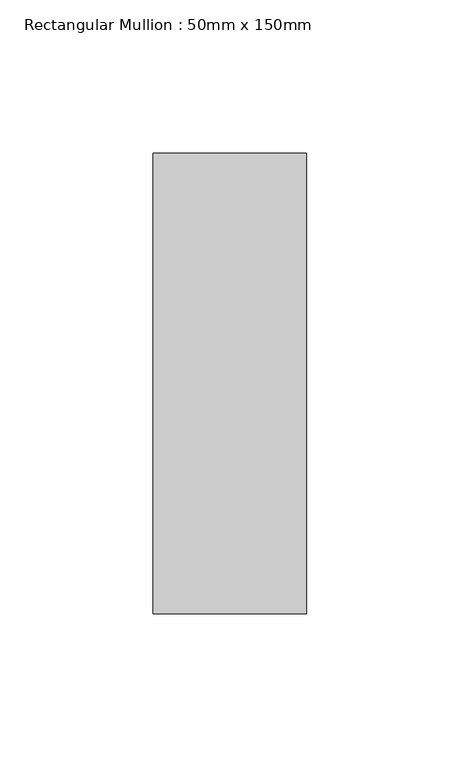
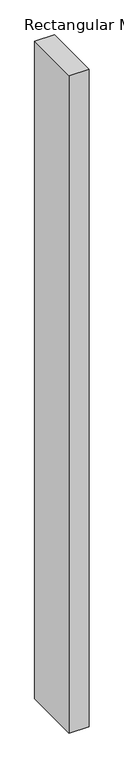
"""IFC4 building model written with IfcOpenShell, lengths in millimetres: member geometry, Rectangular Mullion : 50mm x 150mm."""

from ifc_helpers import new_model, si_unit, frame, origin, place, context, project, spatial, polyline, outline, extrude, source, transform, mapped, element, save


def rectangular_mullion_50mm_x_150mm_ca25adf9(model_context):
    return source(origin(), model_context, "Body", "SweptSolid", [
        extrude(outline(polyline([(25.0, 75.0), (25.0, -75.0), (-25.0, -75.0), (-25.0, 75.0), (25.0, 75.0)])), frame((0.0, 0.0, -1749.4222628), z_axis=(0.0, 0.0, 1.0), x_axis=(1.0, 0.0, 0.0)), (0.0, 0.0, 1.0), 1749.4222628),
    ])


if __name__ == "__main__":
    model = new_model("IFC4")
    model_context = context("Model", 3, world=origin())
    ifc_project = project(units=[si_unit("LENGTHUNIT", "METRE", prefix="MILLI")], contexts=[model_context])
    site = spatial("IfcSite", under=ifc_project)
    building = spatial("IfcBuilding", under=site)
    placement = place(None, origin())
    rectangular_mullion_50mm_x_150mm_shape = rectangular_mullion_50mm_x_150mm_ca25adf9(model_context)
    element("IfcMember", 1, ObjectType="Rectangular Mullion : 50mm x 150mm", at=placement, inside=building, context=model_context, shape_type="MappedRepresentation", body=[
        mapped(rectangular_mullion_50mm_x_150mm_shape, transform((0.0, 0.0, 0.0), x_axis=(1.0, 0.0, 0.0), y_axis=(0.0, 1.0, 0.0), z_axis=(0.0, 0.0, 1.0))),
    ])
    save(model, "model.ifc")

# Revit data of these elements
# Type "Rectangular Mullion : 50mm x 150mm"
#   built-in parameter 1007304 = 0.492126 (stored number, unit not read)
#   built-in parameter 1007301 = 0.082021 (stored number, unit not read)
#   built-in parameter 1007300 = 0.082021 (stored number, unit not read)
# Element 1 (IfcMember, "Rectangular Mullion : 50mm x 150mm")
#   Materials on its faces: "Aluminum"
# Materials
#   "Aluminum": class "Metal", colour RGB 244 244 244, transparency 0, Description = "Aluminum 6061", Cost = 0
